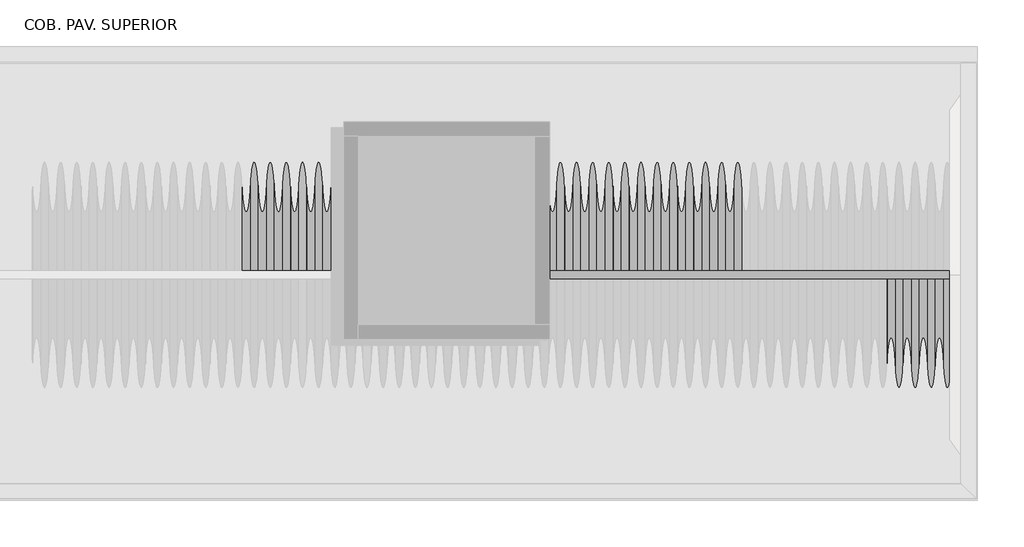
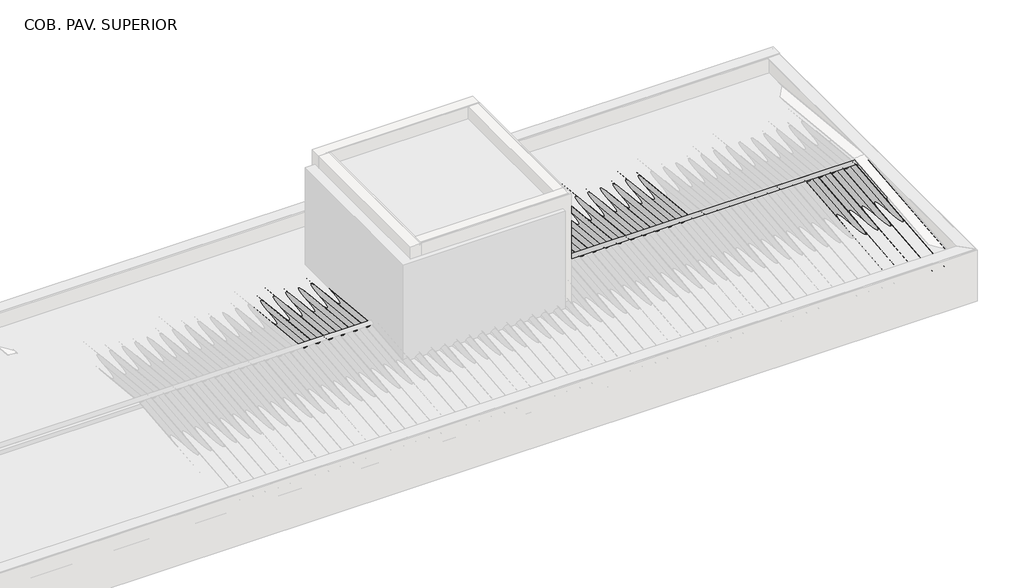
# One storey, part 7 of 8: 46 beams, 8 columns.
"""IFC4 building model written with IfcOpenShell, lengths in millimetres."""

import ifcopenshell
import ifcopenshell.guid

model = None  # the IFC model being written
_history = None  # IfcOwnerHistory: only IFC2X3 demands one
_inside = {}  # id of a spatial element -> (the spatial element, [elements in it])
_under = {}  # id of a project, library or spatial element -> (it, [spatial elements below it])
_declared = {}  # id of a project -> (the project, [libraries it declares])
_typed = {}  # id of a type object -> (the type object, [elements of that type])
_made_of = {}  # id of a material, layer set ... -> (it, [elements and type objects made of it])


def new_model(schema):
    """Start an empty IFC model of exactly this schema.

    Asked for "IFC4X3", IfcOpenShell would pick the latest addendum, in which some entities
    have other attributes; the version numbers below select the first issue.
    IFC2X3 requires an IfcOwnerHistory on every rooted entity: one is made here for all.
    """
    global model, _history
    if schema == "IFC4X3":
        model = ifcopenshell.file(schema_version=(4, 3, 0, 0))
    else:
        model = ifcopenshell.file(schema=schema)
    _inside.clear()
    _under.clear()
    _declared.clear()
    _typed.clear()
    _made_of.clear()
    _history = None
    if model.schema == "IFC2X3":
        org = make("IfcOrganization", Name="unknown")
        user = make(
            "IfcPersonAndOrganization",
            ThePerson=make("IfcPerson", FamilyName="unknown"),
            TheOrganization=org,
        )
        app = make(
            "IfcApplication",
            ApplicationDeveloper=org,
            Version="unknown",
            ApplicationFullName="unknown",
            ApplicationIdentifier="unknown",
        )
        _history = make(
            "IfcOwnerHistory",
            OwningUser=user,
            OwningApplication=app,
            ChangeAction="ADDED",
            CreationDate=0,
        )
    return model


def make(cls, **values):
    """One entity of the class cls with the attributes given. An attribute that is None is left unset."""
    return model.create_entity(
        cls, **{name: value for name, value in values.items() if value is not None}
    )


def rooted(cls, **values):
    """An entity with a GlobalId (a new one), such as an element, a storey or a relation."""
    return make(cls, GlobalId=ifcopenshell.guid.new(), OwnerHistory=_history, **values)


def si_unit(unit_type, name, prefix=None):
    """IfcSIUnit, for example si_unit("LENGTHUNIT", "METRE", prefix="MILLI")."""
    return make("IfcSIUnit", UnitType=unit_type, Prefix=prefix, Name=name)


def assignment(units):
    """IfcUnitAssignment: the units of a project."""
    return None if units is None else make("IfcUnitAssignment", Units=units)


def point(xyz):
    """IfcCartesianPoint."""
    return None if xyz is None else make("IfcCartesianPoint", Coordinates=xyz)


def direction(xyz):
    """IfcDirection."""
    return None if xyz is None else make("IfcDirection", DirectionRatios=xyz)


def frame(location, z_axis=None, x_axis=None):
    """IfcAxis2Placement3D, a coordinate frame: its origin and axes. An axis left out is left unset."""
    return make(
        "IfcAxis2Placement3D",
        Location=point(location),
        Axis=direction(z_axis),
        RefDirection=direction(x_axis),
    )


def frame_2d(location, x_axis=None):
    """IfcAxis2Placement2D, a coordinate frame in the plane: its origin and x axis."""
    return make(
        "IfcAxis2Placement2D", Location=point(location), RefDirection=direction(x_axis)
    )


def origin():
    """The frame at (0, 0, 0) with its axes left unset."""
    return frame((0.0, 0.0, 0.0))


def place(relative_to, where):
    """IfcLocalPlacement: puts the frame where relative to a parent placement (None: the world)."""
    return make(
        "IfcLocalPlacement", PlacementRelTo=relative_to, RelativePlacement=where
    )


def context(
    kind, dimensions, precision=None, world=None, true_north=None, identifier=None
):
    """IfcGeometricRepresentationContext, for example the 3D "Model" context."""
    return make(
        "IfcGeometricRepresentationContext",
        ContextIdentifier=identifier,
        ContextType=kind,
        CoordinateSpaceDimension=dimensions,
        Precision=precision,
        WorldCoordinateSystem=world,
        TrueNorth=true_north,
    )


def project(units=None, contexts=None):
    """IfcProject with its units and contexts."""
    return rooted(
        "IfcProject",
        Name="project",
        RepresentationContexts=contexts,
        UnitsInContext=assignment(units),
    )


def spatial(cls, under=None, at=None, **own):
    """A site, building, storey or space (cls), placed at a placement, below another one or the project."""
    s = rooted(cls, ObjectPlacement=at, **own)
    if under is not None:
        _under.setdefault(under.id(), (under, []))[1].append(s)
    return s


def polyline(points):
    """IfcPolyline through the points."""
    return make("IfcPolyline", Points=[point(p) for p in points])


def circle_curve(where, radius):
    """IfcCircle in the frame where."""
    return make("IfcCircle", Position=where, Radius=radius)


def trimmed(basis, trim1, trim2, sense, master):
    """IfcTrimmedCurve: the piece of a basis curve between two trims."""
    return make(
        "IfcTrimmedCurve",
        BasisCurve=basis,
        Trim1=trim1,
        Trim2=trim2,
        SenseAgreement=sense,
        MasterRepresentation=master,
    )


def segment(curve, same_sense, transition):
    """IfcCompositeCurveSegment."""
    return make(
        "IfcCompositeCurveSegment",
        Transition=transition,
        SameSense=same_sense,
        ParentCurve=curve,
    )


def composite_curve(segments, self_intersect=None):
    """IfcCompositeCurve: segments joined end to end."""
    return make("IfcCompositeCurve", Segments=segments, SelfIntersect=self_intersect)


def outline(outer, holes=None, kind="AREA"):
    """IfcArbitraryClosedProfileDef: a profile drawn as a closed curve; with holes, ...WithVoids."""
    if holes is None:
        return make("IfcArbitraryClosedProfileDef", ProfileType=kind, OuterCurve=outer)
    return make(
        "IfcArbitraryProfileDefWithVoids",
        ProfileType=kind,
        OuterCurve=outer,
        InnerCurves=holes,
    )


def extrude(swept, where, along, depth):
    """IfcExtrudedAreaSolid: the profile swept, set in the frame where, extruded along a direction by depth."""
    return make(
        "IfcExtrudedAreaSolid",
        SweptArea=swept,
        Position=where,
        ExtrudedDirection=direction(along),
        Depth=depth,
    )


def shape(context_of_items, identifier, shape_type, items):
    """IfcShapeRepresentation: the items that make up one representation, for example the "Body"."""
    return make(
        "IfcShapeRepresentation",
        ContextOfItems=context_of_items,
        RepresentationIdentifier=identifier,
        RepresentationType=shape_type,
        Items=items,
    )


def source(mapping_origin, context_of_items, identifier, shape_type, items):
    """IfcRepresentationMap: a shape defined once, which mapped items show again and again."""
    return make(
        "IfcRepresentationMap",
        MappingOrigin=mapping_origin,
        MappedRepresentation=shape(context_of_items, identifier, shape_type, items),
    )


def transform(
    local_origin,
    x_axis=None,
    y_axis=None,
    z_axis=None,
    scale=None,
    scale2=None,
    scale3=None,
    uniform=True,
):
    """IfcCartesianTransformationOperator3D, or its non-uniform kind. x_axis, y_axis, z_axis: its Axis1, 2, 3."""
    if uniform:
        return make(
            "IfcCartesianTransformationOperator3D",
            Axis1=direction(x_axis),
            Axis2=direction(y_axis),
            LocalOrigin=point(local_origin),
            Scale=scale,
            Axis3=direction(z_axis),
        )
    return make(
        "IfcCartesianTransformationOperator3DnonUniform",
        Axis1=direction(x_axis),
        Axis2=direction(y_axis),
        LocalOrigin=point(local_origin),
        Scale=scale,
        Axis3=direction(z_axis),
        Scale2=scale2,
        Scale3=scale3,
    )


def mapped(mapping_source, mapping_target):
    """IfcMappedItem: shows the shape of a source again, moved by a transform."""
    return make(
        "IfcMappedItem", MappingSource=mapping_source, MappingTarget=mapping_target
    )


def made_of(thing, what):
    """Note that an element or type object is made of a material, layer set ...; save() writes the relation."""
    if what is not None:
        _made_of.setdefault(what.id(), (what, []))[1].append(thing)
    return thing


def element(
    cls,
    number,
    at=None,
    inside=None,
    cuts=None,
    type_object=None,
    material=None,
    context=None,
    identifier="Body",
    shape_type=None,
    held_by="IfcProductDefinitionShape",
    body=None,
    shapes=None,
    **own,
):
    """One element of the class cls, such as IfcWall. Its Tag is "e" and its number.

    at: its placement. inside: the storey or other place that contains it. cuts: it is an
    opening in that element (IfcRelVoidsElement). A single representation is given by context,
    identifier, shape_type and body (its items); several are given by shapes. held_by: the class
    of the entity that holds the representations. save() writes the other relations.
    """
    e = rooted(cls, Tag="e%d" % number, ObjectPlacement=at, **own)
    if body is not None:
        shapes = [shape(context, identifier, shape_type, body)]
    if shapes is not None:
        e.Representation = make(held_by, Representations=shapes)
    if inside is not None:
        _inside.setdefault(inside.id(), (inside, []))[1].append(e)
    if cuts is not None:
        rooted(
            "IfcRelVoidsElement", RelatingBuildingElement=cuts, RelatedOpeningElement=e
        )
    if type_object is not None:
        _typed.setdefault(type_object.id(), (type_object, []))[1].append(e)
    return made_of(e, material)


def aggregate(whole, parts):
    """IfcRelAggregates: a whole, such as a stair, and the parts it consists of."""
    return rooted("IfcRelAggregates", RelatingObject=whole, RelatedObjects=parts)


def save(model, path):
    """Write the relations noted so far, then the file.

    IfcRelAggregates (storeys below a building ...), IfcRelContainedInSpatialStructure (elements
    in a storey), IfcRelDefinesByType, IfcRelAssociatesMaterial and IfcRelDeclares: one each for
    every whole, place, type object, material and project.
    """
    for whole, parts in _under.values():
        aggregate(whole, parts)
    for where, things in _inside.values():
        rooted(
            "IfcRelContainedInSpatialStructure",
            RelatedElements=things,
            RelatingStructure=where,
        )
    for kind, things in _typed.values():
        rooted("IfcRelDefinesByType", RelatedObjects=things, RelatingType=kind)
    for what, things in _made_of.values():
        rooted("IfcRelAssociatesMaterial", RelatedObjects=things, RelatingMaterial=what)
    for by, libraries in _declared.values():
        rooted("IfcRelDeclares", RelatingContext=by, RelatedDefinitions=libraries)
    model.write(path)


def beam_fe4ddbad(model_context):
    return source(origin(), model_context, "Body", "SweptSolid", [
        extrude(outline(polyline([(998.8971968, 30.0), (998.8971968, -30.0), (-998.8971974, -30.0), (-998.8971974, 30.0), (998.8971968, 30.0)])), frame((0.0, 0.0, -60.0), z_axis=(0.0, 0.0, 1.0), x_axis=(1.0, 0.0, 0.0)), (0.0, 0.0, 1.0), 120.0),
    ])


def beam_14fb2a3a(model_context):
    return source(origin(), model_context, "Body", "SweptSolid", [
        extrude(outline(polyline([(90.6640427, 30.0), (90.6640427, -30.0), (-90.6640427, -30.0), (-90.6640427, 30.0), (90.6640427, 30.0)])), frame((0.0, 0.0, -60.0), z_axis=(0.0, 0.0, 1.0), x_axis=(1.0, 0.0, 0.0)), (0.0, 0.0, 1.0), 120.0),
    ])


def beam_531541e1(model_context):
    return source(origin(), model_context, "Body", "SweptSolid", [
        extrude(outline(polyline([(789.5608169, 30.0), (789.5608169, -30.0), (-789.5608169, -30.0), (-789.5608169, 30.0), (789.5608169, 30.0)])), frame((0.0, 0.0, -60.0), z_axis=(0.0, 0.0, 1.0), x_axis=(1.0, 0.0, 0.0)), (0.0, 0.0, 1.0), 120.0),
    ])


def cumeeira_telha_ondulada_fibrocimento_e54732c7(model_context):
    return source(origin(), model_context, "Body", "SweptSolid", [
        extrude(outline(composite_curve([segment(polyline([(58.3970135, 42.4437972), (53.9055884, 40.2467307)]), True, "CONTINUOUS"), segment(trimmed(circle_curve(frame_2d((-1.6029865, 13.0936483)), 61.7939461), [point((53.9055884, 40.2467307))], [point((-57.1115615, 40.2467307))], True, "CARTESIAN"), True, "CONTINUOUS"), segment(polyline([(-57.1115615, 40.2467307), (-61.6029865, 42.4437972)]), True, "CONTINUOUS"), segment(trimmed(circle_curve(frame_2d((-1.6029865, 13.0936483)), 66.7939461), [point((-61.6029865, 42.4437972))], [point((58.3970135, 42.4437972))], False, "CARTESIAN"), True, "CONTINUOUS")], self_intersect=False)), frame((-3133.4781794, 0.0, 0.0), z_axis=(1.0, 0.0, 0.0), x_axis=(0.0, 1.0, 0.0)), (0.0, 0.0, 1.0), 6266.9563589),
    ])


def telha_ondulada_fibrocimento_963230a9(model_context):
    return source(origin(), model_context, "Body", "SweptSolid", [
        extrude(outline(composite_curve([segment(trimmed(circle_curve(frame_2d((68.3970135, 71.7939461)), 66.7939461), [point((8.3970135, 42.4437972))], [point((128.3970135, 42.4437972))], True, "CARTESIAN"), True, "CONTINUOUS"), segment(polyline([(128.3970135, 42.4437972), (132.8884385, 40.2467307)]), True, "CONTINUOUS"), segment(trimmed(circle_curve(frame_2d((68.3970135, 71.7939461)), 71.7939461), [point((132.8884385, 40.2467307))], [point((3.9055884, 40.2467307))], False, "CARTESIAN"), True, "CONTINUOUS"), segment(trimmed(circle_curve(frame_2d((-51.6029865, 13.0936483)), 61.7939461), [point((3.9055884, 40.2467307))], [point((-107.1115615, 40.2467307))], True, "CARTESIAN"), True, "CONTINUOUS"), segment(polyline([(-107.1115615, 40.2467307), (-111.6029865, 42.4437972)]), True, "CONTINUOUS"), segment(trimmed(circle_curve(frame_2d((-51.6029865, 13.0936483)), 66.7939461), [point((-111.6029865, 42.4437972))], [point((8.3970135, 42.4437972))], False, "CARTESIAN"), True, "CONTINUOUS")], self_intersect=False)), frame((-362.9289365, 0.0, 0.0), z_axis=(1.0, 0.0, 0.0), x_axis=(0.0, 1.0, 0.0)), (0.0, 0.0, 1.0), 725.8578731),
    ])


def viga_cumeeira_6x16cm_e360fa9d(model_context):
    return source(origin(), model_context, "Body", "SweptSolid", [
        extrude(outline(polyline([(3133.5, 30.0), (3133.5, -30.0), (-3133.5, -30.0), (-3133.5, 30.0), (3133.5, 30.0)])), frame((0.0, 0.0, -80.0), z_axis=(0.0, 0.0, 1.0), x_axis=(1.0, 0.0, 0.0)), (0.0, 0.0, 1.0), 160.0),
    ])


def column_6c15bf79(model_context):
    return source(origin(), model_context, "Body", "SweptSolid", [
        extrude(outline(polyline([(30.0, 80.0), (30.0, -80.0), (-30.0, -80.0), (-30.0, 80.0), (30.0, 80.0)])), frame((0.0, 0.0, 6710.0), z_axis=(0.0, 0.0, 1.0), x_axis=(1.0, 0.0, 0.0)), (0.0, 0.0, 1.0), 467.5),
    ])


def column_910cb117(model_context):
    return source(origin(), model_context, "Body", "SweptSolid", [
        extrude(outline(polyline([(30.0, 80.0), (30.0, -80.0), (-30.0, -80.0), (-30.0, 80.0), (30.0, 80.0)])), frame((0.0, 0.0, 6710.0), z_axis=(0.0, 0.0, 1.0), x_axis=(1.0, 0.0, 0.0)), (0.0, 0.0, 1.0), 371.3),
    ])


def column_42eef9f8(model_context):
    return source(origin(), model_context, "Body", "SweptSolid", [
        extrude(outline(polyline([(30.0, 80.0), (30.0, -80.0), (-30.0, -80.0), (-30.0, 80.0), (30.0, 80.0)])), frame((0.0, 0.0, 6710.0), z_axis=(0.0, 0.0, 1.0), x_axis=(1.0, 0.0, 0.0)), (0.0, 0.0, 1.0), 227.1),
    ])


model = new_model("IFC4")

# Units and contexts
model_context = context("Model", 3, world=origin())
ifc_project = project(units=[si_unit("LENGTHUNIT", "METRE", prefix="MILLI")], contexts=[model_context])

# Site, building, storey
site = spatial("IfcSite", under=ifc_project)
building = spatial("IfcBuilding", under=site)
storey = spatial("IfcBuildingStorey", under=building, Name="COB. PAV. SUPERIOR", Elevation=6650.0)

# Beams
placement = place(None, origin())
beam_shape = beam_fe4ddbad(model_context)
element("IfcBeam", 1, ObjectType="Madeira de lei : Berço 6x12cm", at=placement, inside=storey, context=model_context, shape_type="MappedRepresentation", body=[
    mapped(beam_shape, transform((5549.6158904, -7777.6209418, 6680.0), x_axis=(1.0, 0.0, 0.0), y_axis=(0.0, 0.0, -1.0), z_axis=(0.0, 1.0, 0.0))),
])
element("IfcBeam", 2, ObjectType="Madeira de lei : Berço 6x12cm", at=placement, inside=storey, context=model_context, shape_type="MappedRepresentation", body=[
    mapped(beam_shape, transform((5549.6158904, -6365.3711004, 6680.0), x_axis=(1.0, 0.0, 0.0), y_axis=(0.0, 0.0, -1.0), z_axis=(0.0, 1.0, 0.0))),
])
element("IfcBeam", 3, ObjectType="Madeira de lei : Berço 6x12cm", at=placement, inside=storey, context=model_context, shape_type="MappedRepresentation", body=[
    mapped(beam_shape, transform((7547.4102853, -7777.6209418, 6680.0), x_axis=(1.0, 0.0, 0.0), y_axis=(0.0, 0.0, -1.0), z_axis=(0.0, 1.0, 0.0))),
])
element("IfcBeam", 4, ObjectType="Madeira de lei : Berço 6x12cm", at=placement, inside=storey, context=model_context, shape_type="MappedRepresentation", body=[
    mapped(beam_shape, transform((248.5822594, -7777.6209418, 6680.0), x_axis=(1.0, 0.0, 0.0), y_axis=(0.0, 0.0, -1.0), z_axis=(0.0, 1.0, 0.0))),
])
element("IfcBeam", 5, ObjectType="Madeira de lei : Berço 6x12cm", at=placement, inside=storey, context=model_context, shape_type="MappedRepresentation", body=[
    mapped(beam_shape, transform((248.5822594, -6365.3711004, 6680.0), x_axis=(1.0, 0.0, 0.0), y_axis=(0.0, 0.0, -1.0), z_axis=(0.0, 1.0, 0.0))),
])
element("IfcBeam", 6, ObjectType="Madeira de lei : Berço 6x12cm", at=placement, inside=storey, context=model_context, shape_type="MappedRepresentation", body=[
    mapped(beam_shape, transform((2246.3766557, -4923.3211004, 6680.0), x_axis=(1.0, 0.0, 0.0), y_axis=(0.0, 0.0, -1.0), z_axis=(0.0, 1.0, 0.0))),
])
element("IfcBeam", 7, ObjectType="Madeira de lei : Berço 6x12cm", at=placement, inside=storey, context=model_context, shape_type="MappedRepresentation", body=[
    mapped(beam_shape, transform((248.5822615, -4923.3211004, 6680.0), x_axis=(1.0, 0.0, 0.0), y_axis=(0.0, 0.0, -1.0), z_axis=(0.0, 1.0, 0.0))),
])
beam_2_shape = beam_14fb2a3a(model_context)
element("IfcBeam", 8, ObjectType="Madeira de lei : Berço 6x12cm", at=placement, inside=storey, context=model_context, shape_type="MappedRepresentation", body=[
    mapped(beam_2_shape, transform((1338.1434995, -7777.6209418, 6680.0), x_axis=(1.0, 0.0, 0.0), y_axis=(0.0, 0.0, -1.0), z_axis=(0.0, 1.0, 0.0))),
])
element("IfcBeam", 9, ObjectType="Madeira de lei : Berço 6x12cm", at=placement, inside=storey, context=model_context, shape_type="MappedRepresentation", body=[
    mapped(beam_2_shape, transform((1338.1434995, -6365.3711004, 6680.0), x_axis=(1.0, 0.0, 0.0), y_axis=(0.0, 0.0, -1.0), z_axis=(0.0, 1.0, 0.0))),
])
beam_3_shape = beam_531541e1(model_context)
element("IfcBeam", 10, ObjectType="Madeira de lei : Berço 6x12cm", at=placement, inside=storey, context=model_context, shape_type="MappedRepresentation", body=[
    mapped(beam_3_shape, transform((10028.217853, -9189.768869, 6680.0), x_axis=(1.0, 0.0, 0.0), y_axis=(0.0, 0.0, -1.0), z_axis=(0.0, 1.0, 0.0))),
])
cumeeira_telha_ondulada_fibrocimento_shape = cumeeira_telha_ondulada_fibrocimento_e54732c7(model_context)
element("IfcBeam", 11, ObjectType="Cumeeira Telha Ondulada : Fibrocimento", at=placement, inside=storey, context=model_context, shape_type="MappedRepresentation", body=[
    mapped(cumeeira_telha_ondulada_fibrocimento_shape, transform((7684.2405136, -7777.6209418, 7375.6251229), x_axis=(-1.0, 0.0, 0.0), y_axis=(0.0, -1.0, 0.0), z_axis=(0.0, 0.0, 1.0))),
])
element("IfcBeam", 12, ObjectType="Telha Ondulada : Fibrocimento", at=placement, inside=storey, context=model_context, shape_type="SweptSolid", body=[
    extrude(outline(composite_curve([segment(trimmed(circle_curve(frame_2d((0.0, 66.7939461)), 66.7939461), [point((29.3501489, 6.7939461))], [point((29.3501489, 126.7939461))], True, "CARTESIAN"), True, "CONTINUOUS"), segment(polyline([(29.3501489, 126.7939461), (31.5472154, 131.2853711)]), True, "CONTINUOUS"), segment(trimmed(circle_curve(frame_2d((0.0, 66.7939461)), 71.7939461), [point((31.5472154, 131.2853711))], [point((31.5472154, 2.3025211))], False, "CARTESIAN"), True, "CONTINUOUS"), segment(trimmed(circle_curve(frame_2d((58.7002978, -53.2060539)), 61.7939461), [point((31.5472154, 2.3025211))], [point((31.5472154, -108.7146289))], True, "CARTESIAN"), True, "CONTINUOUS"), segment(polyline([(31.5472154, -108.7146289), (29.3501489, -113.2060539)]), True, "CONTINUOUS"), segment(trimmed(circle_curve(frame_2d((58.7002978, -53.2060539)), 66.7939461), [point((29.3501489, -113.2060539))], [point((29.3501489, 6.7939461))], False, "CARTESIAN"), True, "CONTINUOUS")], self_intersect=False)), frame((9796.7156257, -10831.9594023, 7106.8215886), z_axis=(0.0, 0.9950371902099894, 0.09950371902099749), x_axis=(0.0, 0.09950371902099749, -0.9950371902099894)), (0.0, 0.0, 1.0), 3060.4439799),
])
element("IfcBeam", 13, ObjectType="Telha Ondulada : Fibrocimento", at=placement, inside=storey, context=model_context, shape_type="SweptSolid", body=[
    extrude(outline(composite_curve([segment(trimmed(circle_curve(frame_2d((0.0, 66.7939461)), 66.7939461), [point((29.3501489, 6.7939461))], [point((29.3501489, 126.7939461))], True, "CARTESIAN"), True, "CONTINUOUS"), segment(polyline([(29.3501489, 126.7939461), (31.5472154, 131.2853711)]), True, "CONTINUOUS"), segment(trimmed(circle_curve(frame_2d((0.0, 66.7939461)), 71.7939461), [point((31.5472154, 131.2853711))], [point((31.5472154, 2.3025211))], False, "CARTESIAN"), True, "CONTINUOUS"), segment(trimmed(circle_curve(frame_2d((58.7002978, -53.2060539)), 61.7939461), [point((31.5472154, 2.3025211))], [point((31.5472154, -108.7146289))], True, "CARTESIAN"), True, "CONTINUOUS"), segment(polyline([(31.5472154, -108.7146289), (29.3501489, -113.2060539)]), True, "CONTINUOUS"), segment(trimmed(circle_curve(frame_2d((58.7002978, -53.2060539)), 66.7939461), [point((29.3501489, -113.2060539))], [point((29.3501489, 6.7939461))], False, "CARTESIAN"), True, "CONTINUOUS")], self_intersect=False)), frame((10041.2156257, -10831.9594023, 7106.8215886), z_axis=(0.0, 0.9950371902099894, 0.09950371902099749), x_axis=(0.0, 0.09950371902099749, -0.9950371902099894)), (0.0, 0.0, 1.0), 3060.4439799),
])
element("IfcBeam", 14, ObjectType="Telha Ondulada : Fibrocimento", at=placement, inside=storey, context=model_context, shape_type="SweptSolid", body=[
    extrude(outline(composite_curve([segment(trimmed(circle_curve(frame_2d((0.0, 66.7939461)), 66.7939461), [point((29.3501489, 6.7939461))], [point((29.3501489, 126.7939461))], True, "CARTESIAN"), True, "CONTINUOUS"), segment(polyline([(29.3501489, 126.7939461), (31.5472154, 131.2853711)]), True, "CONTINUOUS"), segment(trimmed(circle_curve(frame_2d((0.0, 66.7939461)), 71.7939461), [point((31.5472154, 131.2853711))], [point((31.5472154, 2.3025211))], False, "CARTESIAN"), True, "CONTINUOUS"), segment(trimmed(circle_curve(frame_2d((58.7002978, -53.2060539)), 61.7939461), [point((31.5472154, 2.3025211))], [point((31.5472154, -108.7146289))], True, "CARTESIAN"), True, "CONTINUOUS"), segment(polyline([(31.5472154, -108.7146289), (29.3501489, -113.2060539)]), True, "CONTINUOUS"), segment(trimmed(circle_curve(frame_2d((58.7002978, -53.2060539)), 66.7939461), [point((29.3501489, -113.2060539))], [point((29.3501489, 6.7939461))], False, "CARTESIAN"), True, "CONTINUOUS")], self_intersect=False)), frame((10285.7156257, -10831.9594023, 7106.8215886), z_axis=(0.0, 0.9950371902099894, 0.09950371902099749), x_axis=(0.0, 0.09950371902099749, -0.9950371902099894)), (0.0, 0.0, 1.0), 3060.4439799),
])
element("IfcBeam", 15, ObjectType="Telha Ondulada : Fibrocimento", at=placement, inside=storey, context=model_context, shape_type="SweptSolid", body=[
    extrude(outline(composite_curve([segment(trimmed(circle_curve(frame_2d((0.0, 66.7939461)), 66.7939461), [point((29.3501489, 6.7939461))], [point((29.3501489, 126.7939461))], True, "CARTESIAN"), True, "CONTINUOUS"), segment(polyline([(29.3501489, 126.7939461), (31.5472154, 131.2853711)]), True, "CONTINUOUS"), segment(trimmed(circle_curve(frame_2d((0.0, 66.7939461)), 71.7939461), [point((31.5472154, 131.2853711))], [point((31.5472154, 2.3025211))], False, "CARTESIAN"), True, "CONTINUOUS"), segment(trimmed(circle_curve(frame_2d((58.7002978, -53.2060539)), 61.7939461), [point((31.5472154, 2.3025211))], [point((31.5472154, -108.7146289))], True, "CARTESIAN"), True, "CONTINUOUS"), segment(polyline([(31.5472154, -108.7146289), (29.3501489, -113.2060539)]), True, "CONTINUOUS"), segment(trimmed(circle_curve(frame_2d((58.7002978, -53.2060539)), 66.7939461), [point((29.3501489, -113.2060539))], [point((29.3501489, 6.7939461))], False, "CARTESIAN"), True, "CONTINUOUS")], self_intersect=False)), frame((10530.2156257, -10831.9594023, 7106.8215886), z_axis=(0.0, 0.9950371902099894, 0.09950371902099749), x_axis=(0.0, 0.09950371902099749, -0.9950371902099894)), (0.0, 0.0, 1.0), 3060.4439799),
])
element("IfcBeam", 16, ObjectType="Telha Ondulada : Fibrocimento", at=placement, inside=storey, context=model_context, shape_type="SweptSolid", body=[
    extrude(outline(composite_curve([segment(trimmed(circle_curve(frame_2d((0.0, 66.7939461)), 66.7939461), [point((29.3501489, 6.7939461))], [point((29.3501489, 126.7939461))], True, "CARTESIAN"), True, "CONTINUOUS"), segment(polyline([(29.3501489, 126.7939461), (31.5472154, 131.2853711)]), True, "CONTINUOUS"), segment(trimmed(circle_curve(frame_2d((0.0, 66.7939461)), 71.7939461), [point((31.5472154, 131.2853711))], [point((31.5472154, 2.3025211))], False, "CARTESIAN"), True, "CONTINUOUS"), segment(trimmed(circle_curve(frame_2d((58.7002978, -53.2060539)), 61.7939461), [point((31.5472154, 2.3025211))], [point((31.5472154, -108.7146289))], True, "CARTESIAN"), True, "CONTINUOUS"), segment(polyline([(31.5472154, -108.7146289), (29.3501489, -113.2060539)]), True, "CONTINUOUS"), segment(trimmed(circle_curve(frame_2d((58.7002978, -53.2060539)), 66.7939461), [point((29.3501489, -113.2060539))], [point((29.3501489, 6.7939461))], False, "CARTESIAN"), True, "CONTINUOUS")], self_intersect=False)), frame((10774.7156257, -10831.9594023, 7106.8215886), z_axis=(0.0, 0.9950371902099894, 0.09950371902099749), x_axis=(0.0, 0.09950371902099749, -0.9950371902099894)), (0.0, 0.0, 1.0), 3060.4439799),
])
element("IfcBeam", 17, ObjectType="Telha Ondulada : Fibrocimento", at=placement, inside=storey, context=model_context, shape_type="SweptSolid", body=[
    extrude(outline(composite_curve([segment(trimmed(circle_curve(frame_2d((-58.7002978, -53.2060539)), 66.7939461), [point((-29.3501489, 6.7939461))], [point((-29.3501489, -113.2060539))], False, "CARTESIAN"), True, "CONTINUOUS"), segment(polyline([(-29.3501489, -113.2060539), (-31.5472154, -108.7146289)]), True, "CONTINUOUS"), segment(trimmed(circle_curve(frame_2d((-58.7002978, -53.2060539)), 61.7939461), [point((-31.5472154, -108.7146289))], [point((-31.5472154, 2.3025211))], True, "CARTESIAN"), True, "CONTINUOUS"), segment(trimmed(circle_curve(frame_2d((0.0, 66.7939461)), 71.7939461), [point((-31.5472154, 2.3025211))], [point((-31.5472154, 131.2853711))], False, "CARTESIAN"), True, "CONTINUOUS"), segment(polyline([(-31.5472154, 131.2853711), (-29.3501489, 126.7939461)]), True, "CONTINUOUS"), segment(trimmed(circle_curve(frame_2d((0.0, 66.7939461)), 66.7939461), [point((-29.3501489, 126.7939461))], [point((-29.3501489, 6.7939461))], True, "CARTESIAN"), True, "CONTINUOUS")], self_intersect=False)), frame((16.7156257, -4723.1805671, 7106.8215886), z_axis=(0.0, -0.9950371902099893, 0.09950371902099796), x_axis=(0.0, 0.09950371902099796, 0.9950371902099893)), (0.0, 0.0, 1.0), 3060.4439799),
])
element("IfcBeam", 18, ObjectType="Telha Ondulada : Fibrocimento", at=placement, inside=storey, context=model_context, shape_type="SweptSolid", body=[
    extrude(outline(composite_curve([segment(trimmed(circle_curve(frame_2d((-58.7002978, -53.2060539)), 66.7939461), [point((-29.3501489, 6.7939461))], [point((-29.3501489, -113.2060539))], False, "CARTESIAN"), True, "CONTINUOUS"), segment(polyline([(-29.3501489, -113.2060539), (-31.5472154, -108.7146289)]), True, "CONTINUOUS"), segment(trimmed(circle_curve(frame_2d((-58.7002978, -53.2060539)), 61.7939461), [point((-31.5472154, -108.7146289))], [point((-31.5472154, 2.3025211))], True, "CARTESIAN"), True, "CONTINUOUS"), segment(trimmed(circle_curve(frame_2d((0.0, 66.7939461)), 71.7939461), [point((-31.5472154, 2.3025211))], [point((-31.5472154, 131.2853711))], False, "CARTESIAN"), True, "CONTINUOUS"), segment(polyline([(-31.5472154, 131.2853711), (-29.3501489, 126.7939461)]), True, "CONTINUOUS"), segment(trimmed(circle_curve(frame_2d((0.0, 66.7939461)), 66.7939461), [point((-29.3501489, 126.7939461))], [point((-29.3501489, 6.7939461))], True, "CARTESIAN"), True, "CONTINUOUS")], self_intersect=False)), frame((261.2156257, -4723.1805671, 7106.8215886), z_axis=(0.0, -0.9950371902099893, 0.09950371902099796), x_axis=(0.0, 0.09950371902099796, 0.9950371902099893)), (0.0, 0.0, 1.0), 3060.4439799),
])
element("IfcBeam", 19, ObjectType="Telha Ondulada : Fibrocimento", at=placement, inside=storey, context=model_context, shape_type="SweptSolid", body=[
    extrude(outline(composite_curve([segment(trimmed(circle_curve(frame_2d((-58.7002978, -53.2060539)), 66.7939461), [point((-29.3501489, 6.7939461))], [point((-29.3501489, -113.2060539))], False, "CARTESIAN"), True, "CONTINUOUS"), segment(polyline([(-29.3501489, -113.2060539), (-31.5472154, -108.7146289)]), True, "CONTINUOUS"), segment(trimmed(circle_curve(frame_2d((-58.7002978, -53.2060539)), 61.7939461), [point((-31.5472154, -108.7146289))], [point((-31.5472154, 2.3025211))], True, "CARTESIAN"), True, "CONTINUOUS"), segment(trimmed(circle_curve(frame_2d((0.0, 66.7939461)), 71.7939461), [point((-31.5472154, 2.3025211))], [point((-31.5472154, 131.2853711))], False, "CARTESIAN"), True, "CONTINUOUS"), segment(polyline([(-31.5472154, 131.2853711), (-29.3501489, 126.7939461)]), True, "CONTINUOUS"), segment(trimmed(circle_curve(frame_2d((0.0, 66.7939461)), 66.7939461), [point((-29.3501489, 126.7939461))], [point((-29.3501489, 6.7939461))], True, "CARTESIAN"), True, "CONTINUOUS")], self_intersect=False)), frame((505.7156257, -4723.1805671, 7106.8215886), z_axis=(0.0, -0.9950371902099893, 0.09950371902099796), x_axis=(0.0, 0.09950371902099796, 0.9950371902099893)), (0.0, 0.0, 1.0), 3060.4439799),
])
element("IfcBeam", 20, ObjectType="Telha Ondulada : Fibrocimento", at=placement, inside=storey, context=model_context, shape_type="SweptSolid", body=[
    extrude(outline(composite_curve([segment(trimmed(circle_curve(frame_2d((-58.7002978, -53.2060539)), 66.7939461), [point((-29.3501489, 6.7939461))], [point((-29.3501489, -113.2060539))], False, "CARTESIAN"), True, "CONTINUOUS"), segment(polyline([(-29.3501489, -113.2060539), (-31.5472154, -108.7146289)]), True, "CONTINUOUS"), segment(trimmed(circle_curve(frame_2d((-58.7002978, -53.2060539)), 61.7939461), [point((-31.5472154, -108.7146289))], [point((-31.5472154, 2.3025211))], True, "CARTESIAN"), True, "CONTINUOUS"), segment(trimmed(circle_curve(frame_2d((0.0, 66.7939461)), 71.7939461), [point((-31.5472154, 2.3025211))], [point((-31.5472154, 131.2853711))], False, "CARTESIAN"), True, "CONTINUOUS"), segment(polyline([(-31.5472154, 131.2853711), (-29.3501489, 126.7939461)]), True, "CONTINUOUS"), segment(trimmed(circle_curve(frame_2d((0.0, 66.7939461)), 66.7939461), [point((-29.3501489, 126.7939461))], [point((-29.3501489, 6.7939461))], True, "CARTESIAN"), True, "CONTINUOUS")], self_intersect=False)), frame((750.2156257, -4723.1805671, 7106.8215886), z_axis=(0.0, -0.9950371902099893, 0.09950371902099796), x_axis=(0.0, 0.09950371902099796, 0.9950371902099893)), (0.0, 0.0, 1.0), 3060.4439799),
])
element("IfcBeam", 21, ObjectType="Telha Ondulada : Fibrocimento", at=placement, inside=storey, context=model_context, shape_type="SweptSolid", body=[
    extrude(outline(composite_curve([segment(trimmed(circle_curve(frame_2d((-58.7002978, -53.2060539)), 66.7939461), [point((-29.3501489, 6.7939461))], [point((-29.3501489, -113.2060539))], False, "CARTESIAN"), True, "CONTINUOUS"), segment(polyline([(-29.3501489, -113.2060539), (-31.5472154, -108.7146289)]), True, "CONTINUOUS"), segment(trimmed(circle_curve(frame_2d((-58.7002978, -53.2060539)), 61.7939461), [point((-31.5472154, -108.7146289))], [point((-31.5472154, 2.3025211))], True, "CARTESIAN"), True, "CONTINUOUS"), segment(trimmed(circle_curve(frame_2d((0.0, 66.7939461)), 71.7939461), [point((-31.5472154, 2.3025211))], [point((-31.5472154, 131.2853711))], False, "CARTESIAN"), True, "CONTINUOUS"), segment(polyline([(-31.5472154, 131.2853711), (-29.3501489, 126.7939461)]), True, "CONTINUOUS"), segment(trimmed(circle_curve(frame_2d((0.0, 66.7939461)), 66.7939461), [point((-29.3501489, 126.7939461))], [point((-29.3501489, 6.7939461))], True, "CARTESIAN"), True, "CONTINUOUS")], self_intersect=False)), frame((994.7156257, -4723.1805671, 7106.8215886), z_axis=(0.0, -0.9950371902099893, 0.09950371902099796), x_axis=(0.0, 0.09950371902099796, 0.9950371902099893)), (0.0, 0.0, 1.0), 3060.4439799),
])
element("IfcBeam", 22, ObjectType="Telha Ondulada : Fibrocimento", at=placement, inside=storey, context=model_context, shape_type="SweptSolid", body=[
    extrude(outline(composite_curve([segment(trimmed(circle_curve(frame_2d((-58.7002978, -53.2060539)), 66.7939461), [point((-29.3501489, 6.7939461))], [point((-29.3501489, -113.2060539))], False, "CARTESIAN"), True, "CONTINUOUS"), segment(polyline([(-29.3501489, -113.2060539), (-31.5472154, -108.7146289)]), True, "CONTINUOUS"), segment(trimmed(circle_curve(frame_2d((-58.7002978, -53.2060539)), 61.7939461), [point((-31.5472154, -108.7146289))], [point((-31.5472154, 2.3025211))], True, "CARTESIAN"), True, "CONTINUOUS"), segment(trimmed(circle_curve(frame_2d((0.0, 66.7939461)), 71.7939461), [point((-31.5472154, 2.3025211))], [point((-31.5472154, 131.2853711))], False, "CARTESIAN"), True, "CONTINUOUS"), segment(polyline([(-31.5472154, 131.2853711), (-29.3501489, 126.7939461)]), True, "CONTINUOUS"), segment(trimmed(circle_curve(frame_2d((0.0, 66.7939461)), 66.7939461), [point((-29.3501489, 126.7939461))], [point((-29.3501489, 6.7939461))], True, "CARTESIAN"), True, "CONTINUOUS")], self_intersect=False)), frame((1239.2156257, -4723.1805671, 7106.8215886), z_axis=(0.0, -0.9950371902099893, 0.09950371902099796), x_axis=(0.0, 0.09950371902099796, 0.9950371902099893)), (0.0, 0.0, 1.0), 3060.4439799),
])
element("IfcBeam", 23, ObjectType="Telha Ondulada : Fibrocimento", at=placement, inside=storey, context=model_context, shape_type="SweptSolid", body=[
    extrude(outline(composite_curve([segment(trimmed(circle_curve(frame_2d((-58.7002978, -53.2060539)), 66.7939461), [point((-29.3501489, 6.7939461))], [point((-29.3501489, -113.2060539))], False, "CARTESIAN"), True, "CONTINUOUS"), segment(polyline([(-29.3501489, -113.2060539), (-31.5472154, -108.7146289)]), True, "CONTINUOUS"), segment(trimmed(circle_curve(frame_2d((-58.7002978, -53.2060539)), 61.7939461), [point((-31.5472154, -108.7146289))], [point((-31.5472154, 2.3025211))], True, "CARTESIAN"), True, "CONTINUOUS"), segment(trimmed(circle_curve(frame_2d((0.0, 66.7939461)), 71.7939461), [point((-31.5472154, 2.3025211))], [point((-31.5472154, 131.2853711))], False, "CARTESIAN"), True, "CONTINUOUS"), segment(polyline([(-31.5472154, 131.2853711), (-29.3501489, 126.7939461)]), True, "CONTINUOUS"), segment(trimmed(circle_curve(frame_2d((0.0, 66.7939461)), 66.7939461), [point((-29.3501489, 126.7939461))], [point((-29.3501489, 6.7939461))], True, "CARTESIAN"), True, "CONTINUOUS")], self_intersect=False)), frame((4662.2156257, -4723.1805671, 7106.8215886), z_axis=(0.0, -0.9950371902099893, 0.09950371902099783), x_axis=(0.0, 0.09950371902099783, 0.9950371902099893)), (0.0, 0.0, 1.0), 3060.4439799),
])
element("IfcBeam", 24, ObjectType="Telha Ondulada : Fibrocimento", at=placement, inside=storey, context=model_context, shape_type="SweptSolid", body=[
    extrude(outline(composite_curve([segment(trimmed(circle_curve(frame_2d((-58.7002978, -53.2060539)), 66.7939461), [point((-29.3501489, 6.7939461))], [point((-29.3501489, -113.2060539))], False, "CARTESIAN"), True, "CONTINUOUS"), segment(polyline([(-29.3501489, -113.2060539), (-31.5472154, -108.7146289)]), True, "CONTINUOUS"), segment(trimmed(circle_curve(frame_2d((-58.7002978, -53.2060539)), 61.7939461), [point((-31.5472154, -108.7146289))], [point((-31.5472154, 2.3025211))], True, "CARTESIAN"), True, "CONTINUOUS"), segment(trimmed(circle_curve(frame_2d((0.0, 66.7939461)), 71.7939461), [point((-31.5472154, 2.3025211))], [point((-31.5472154, 131.2853711))], False, "CARTESIAN"), True, "CONTINUOUS"), segment(polyline([(-31.5472154, 131.2853711), (-29.3501489, 126.7939461)]), True, "CONTINUOUS"), segment(trimmed(circle_curve(frame_2d((0.0, 66.7939461)), 66.7939461), [point((-29.3501489, 126.7939461))], [point((-29.3501489, 6.7939461))], True, "CARTESIAN"), True, "CONTINUOUS")], self_intersect=False)), frame((4906.7156257, -4723.1805671, 7106.8215886), z_axis=(0.0, -0.9950371902099893, 0.09950371902099783), x_axis=(0.0, 0.09950371902099783, 0.9950371902099893)), (0.0, 0.0, 1.0), 3060.4439799),
])
element("IfcBeam", 25, ObjectType="Telha Ondulada : Fibrocimento", at=placement, inside=storey, context=model_context, shape_type="SweptSolid", body=[
    extrude(outline(composite_curve([segment(trimmed(circle_curve(frame_2d((-58.7002978, -53.2060539)), 66.7939461), [point((-29.3501489, 6.7939461))], [point((-29.3501489, -113.2060539))], False, "CARTESIAN"), True, "CONTINUOUS"), segment(polyline([(-29.3501489, -113.2060539), (-31.5472154, -108.7146289)]), True, "CONTINUOUS"), segment(trimmed(circle_curve(frame_2d((-58.7002978, -53.2060539)), 61.7939461), [point((-31.5472154, -108.7146289))], [point((-31.5472154, 2.3025211))], True, "CARTESIAN"), True, "CONTINUOUS"), segment(trimmed(circle_curve(frame_2d((0.0, 66.7939461)), 71.7939461), [point((-31.5472154, 2.3025211))], [point((-31.5472154, 131.2853711))], False, "CARTESIAN"), True, "CONTINUOUS"), segment(polyline([(-31.5472154, 131.2853711), (-29.3501489, 126.7939461)]), True, "CONTINUOUS"), segment(trimmed(circle_curve(frame_2d((0.0, 66.7939461)), 66.7939461), [point((-29.3501489, 126.7939461))], [point((-29.3501489, 6.7939461))], True, "CARTESIAN"), True, "CONTINUOUS")], self_intersect=False)), frame((5151.2156257, -4723.1805671, 7106.8215886), z_axis=(0.0, -0.9950371902099893, 0.09950371902099783), x_axis=(0.0, 0.09950371902099783, 0.9950371902099893)), (0.0, 0.0, 1.0), 3060.4439799),
])
element("IfcBeam", 26, ObjectType="Telha Ondulada : Fibrocimento", at=placement, inside=storey, context=model_context, shape_type="SweptSolid", body=[
    extrude(outline(composite_curve([segment(trimmed(circle_curve(frame_2d((-58.7002978, -53.2060539)), 66.7939461), [point((-29.3501489, 6.7939461))], [point((-29.3501489, -113.2060539))], False, "CARTESIAN"), True, "CONTINUOUS"), segment(polyline([(-29.3501489, -113.2060539), (-31.5472154, -108.7146289)]), True, "CONTINUOUS"), segment(trimmed(circle_curve(frame_2d((-58.7002978, -53.2060539)), 61.7939461), [point((-31.5472154, -108.7146289))], [point((-31.5472154, 2.3025211))], True, "CARTESIAN"), True, "CONTINUOUS"), segment(trimmed(circle_curve(frame_2d((0.0, 66.7939461)), 71.7939461), [point((-31.5472154, 2.3025211))], [point((-31.5472154, 131.2853711))], False, "CARTESIAN"), True, "CONTINUOUS"), segment(polyline([(-31.5472154, 131.2853711), (-29.3501489, 126.7939461)]), True, "CONTINUOUS"), segment(trimmed(circle_curve(frame_2d((0.0, 66.7939461)), 66.7939461), [point((-29.3501489, 126.7939461))], [point((-29.3501489, 6.7939461))], True, "CARTESIAN"), True, "CONTINUOUS")], self_intersect=False)), frame((5395.7156257, -4723.1805671, 7106.8215886), z_axis=(0.0, -0.9950371902099893, 0.09950371902099783), x_axis=(0.0, 0.09950371902099783, 0.9950371902099893)), (0.0, 0.0, 1.0), 3060.4439799),
])
element("IfcBeam", 27, ObjectType="Telha Ondulada : Fibrocimento", at=placement, inside=storey, context=model_context, shape_type="SweptSolid", body=[
    extrude(outline(composite_curve([segment(trimmed(circle_curve(frame_2d((-58.7002978, -53.2060539)), 66.7939461), [point((-29.3501489, 6.7939461))], [point((-29.3501489, -113.2060539))], False, "CARTESIAN"), True, "CONTINUOUS"), segment(polyline([(-29.3501489, -113.2060539), (-31.5472154, -108.7146289)]), True, "CONTINUOUS"), segment(trimmed(circle_curve(frame_2d((-58.7002978, -53.2060539)), 61.7939461), [point((-31.5472154, -108.7146289))], [point((-31.5472154, 2.3025211))], True, "CARTESIAN"), True, "CONTINUOUS"), segment(trimmed(circle_curve(frame_2d((0.0, 66.7939461)), 71.7939461), [point((-31.5472154, 2.3025211))], [point((-31.5472154, 131.2853711))], False, "CARTESIAN"), True, "CONTINUOUS"), segment(polyline([(-31.5472154, 131.2853711), (-29.3501489, 126.7939461)]), True, "CONTINUOUS"), segment(trimmed(circle_curve(frame_2d((0.0, 66.7939461)), 66.7939461), [point((-29.3501489, 126.7939461))], [point((-29.3501489, 6.7939461))], True, "CARTESIAN"), True, "CONTINUOUS")], self_intersect=False)), frame((5640.2156257, -4723.1805671, 7106.8215886), z_axis=(0.0, -0.9950371902099893, 0.09950371902099783), x_axis=(0.0, 0.09950371902099783, 0.9950371902099893)), (0.0, 0.0, 1.0), 3060.4439799),
])
element("IfcBeam", 28, ObjectType="Telha Ondulada : Fibrocimento", at=placement, inside=storey, context=model_context, shape_type="SweptSolid", body=[
    extrude(outline(composite_curve([segment(trimmed(circle_curve(frame_2d((-58.7002978, -53.2060539)), 66.7939461), [point((-29.3501489, 6.7939461))], [point((-29.3501489, -113.2060539))], False, "CARTESIAN"), True, "CONTINUOUS"), segment(polyline([(-29.3501489, -113.2060539), (-31.5472154, -108.7146289)]), True, "CONTINUOUS"), segment(trimmed(circle_curve(frame_2d((-58.7002978, -53.2060539)), 61.7939461), [point((-31.5472154, -108.7146289))], [point((-31.5472154, 2.3025211))], True, "CARTESIAN"), True, "CONTINUOUS"), segment(trimmed(circle_curve(frame_2d((0.0, 66.7939461)), 71.7939461), [point((-31.5472154, 2.3025211))], [point((-31.5472154, 131.2853711))], False, "CARTESIAN"), True, "CONTINUOUS"), segment(polyline([(-31.5472154, 131.2853711), (-29.3501489, 126.7939461)]), True, "CONTINUOUS"), segment(trimmed(circle_curve(frame_2d((0.0, 66.7939461)), 66.7939461), [point((-29.3501489, 126.7939461))], [point((-29.3501489, 6.7939461))], True, "CARTESIAN"), True, "CONTINUOUS")], self_intersect=False)), frame((5884.7156257, -4723.1805671, 7106.8215886), z_axis=(0.0, -0.9950371902099893, 0.09950371902099783), x_axis=(0.0, 0.09950371902099783, 0.9950371902099893)), (0.0, 0.0, 1.0), 3060.4439799),
])
element("IfcBeam", 29, ObjectType="Telha Ondulada : Fibrocimento", at=placement, inside=storey, context=model_context, shape_type="SweptSolid", body=[
    extrude(outline(composite_curve([segment(trimmed(circle_curve(frame_2d((-58.7002978, -53.2060539)), 66.7939461), [point((-29.3501489, 6.7939461))], [point((-29.3501489, -113.2060539))], False, "CARTESIAN"), True, "CONTINUOUS"), segment(polyline([(-29.3501489, -113.2060539), (-31.5472154, -108.7146289)]), True, "CONTINUOUS"), segment(trimmed(circle_curve(frame_2d((-58.7002978, -53.2060539)), 61.7939461), [point((-31.5472154, -108.7146289))], [point((-31.5472154, 2.3025211))], True, "CARTESIAN"), True, "CONTINUOUS"), segment(trimmed(circle_curve(frame_2d((0.0, 66.7939461)), 71.7939461), [point((-31.5472154, 2.3025211))], [point((-31.5472154, 131.2853711))], False, "CARTESIAN"), True, "CONTINUOUS"), segment(polyline([(-31.5472154, 131.2853711), (-29.3501489, 126.7939461)]), True, "CONTINUOUS"), segment(trimmed(circle_curve(frame_2d((0.0, 66.7939461)), 66.7939461), [point((-29.3501489, 126.7939461))], [point((-29.3501489, 6.7939461))], True, "CARTESIAN"), True, "CONTINUOUS")], self_intersect=False)), frame((6129.2156257, -4723.1805671, 7106.8215886), z_axis=(0.0, -0.9950371902099893, 0.09950371902099783), x_axis=(0.0, 0.09950371902099783, 0.9950371902099893)), (0.0, 0.0, 1.0), 3060.4439799),
])
element("IfcBeam", 30, ObjectType="Telha Ondulada : Fibrocimento", at=placement, inside=storey, context=model_context, shape_type="SweptSolid", body=[
    extrude(outline(composite_curve([segment(trimmed(circle_curve(frame_2d((-58.7002978, -53.2060539)), 66.7939461), [point((-29.3501489, 6.7939461))], [point((-29.3501489, -113.2060539))], False, "CARTESIAN"), True, "CONTINUOUS"), segment(polyline([(-29.3501489, -113.2060539), (-31.5472154, -108.7146289)]), True, "CONTINUOUS"), segment(trimmed(circle_curve(frame_2d((-58.7002978, -53.2060539)), 61.7939461), [point((-31.5472154, -108.7146289))], [point((-31.5472154, 2.3025211))], True, "CARTESIAN"), True, "CONTINUOUS"), segment(trimmed(circle_curve(frame_2d((0.0, 66.7939461)), 71.7939461), [point((-31.5472154, 2.3025211))], [point((-31.5472154, 131.2853711))], False, "CARTESIAN"), True, "CONTINUOUS"), segment(polyline([(-31.5472154, 131.2853711), (-29.3501489, 126.7939461)]), True, "CONTINUOUS"), segment(trimmed(circle_curve(frame_2d((0.0, 66.7939461)), 66.7939461), [point((-29.3501489, 126.7939461))], [point((-29.3501489, 6.7939461))], True, "CARTESIAN"), True, "CONTINUOUS")], self_intersect=False)), frame((6373.7156257, -4723.1805671, 7106.8215886), z_axis=(0.0, -0.9950371902099893, 0.09950371902099783), x_axis=(0.0, 0.09950371902099783, 0.9950371902099893)), (0.0, 0.0, 1.0), 3060.4439799),
])
element("IfcBeam", 31, ObjectType="Telha Ondulada : Fibrocimento", at=placement, inside=storey, context=model_context, shape_type="SweptSolid", body=[
    extrude(outline(composite_curve([segment(trimmed(circle_curve(frame_2d((-58.7002978, -53.2060539)), 66.7939461), [point((-29.3501489, 6.7939461))], [point((-29.3501489, -113.2060539))], False, "CARTESIAN"), True, "CONTINUOUS"), segment(polyline([(-29.3501489, -113.2060539), (-31.5472154, -108.7146289)]), True, "CONTINUOUS"), segment(trimmed(circle_curve(frame_2d((-58.7002978, -53.2060539)), 61.7939461), [point((-31.5472154, -108.7146289))], [point((-31.5472154, 2.3025211))], True, "CARTESIAN"), True, "CONTINUOUS"), segment(trimmed(circle_curve(frame_2d((0.0, 66.7939461)), 71.7939461), [point((-31.5472154, 2.3025211))], [point((-31.5472154, 131.2853711))], False, "CARTESIAN"), True, "CONTINUOUS"), segment(polyline([(-31.5472154, 131.2853711), (-29.3501489, 126.7939461)]), True, "CONTINUOUS"), segment(trimmed(circle_curve(frame_2d((0.0, 66.7939461)), 66.7939461), [point((-29.3501489, 126.7939461))], [point((-29.3501489, 6.7939461))], True, "CARTESIAN"), True, "CONTINUOUS")], self_intersect=False)), frame((6618.2156257, -4723.1805671, 7106.8215886), z_axis=(0.0, -0.9950371902099893, 0.09950371902099783), x_axis=(0.0, 0.09950371902099783, 0.9950371902099893)), (0.0, 0.0, 1.0), 3060.4439799),
])
element("IfcBeam", 32, ObjectType="Telha Ondulada : Fibrocimento", at=placement, inside=storey, context=model_context, shape_type="SweptSolid", body=[
    extrude(outline(composite_curve([segment(trimmed(circle_curve(frame_2d((-58.7002978, -53.2060539)), 66.7939461), [point((-29.3501489, 6.7939461))], [point((-29.3501489, -113.2060539))], False, "CARTESIAN"), True, "CONTINUOUS"), segment(polyline([(-29.3501489, -113.2060539), (-31.5472154, -108.7146289)]), True, "CONTINUOUS"), segment(trimmed(circle_curve(frame_2d((-58.7002978, -53.2060539)), 61.7939461), [point((-31.5472154, -108.7146289))], [point((-31.5472154, 2.3025211))], True, "CARTESIAN"), True, "CONTINUOUS"), segment(trimmed(circle_curve(frame_2d((0.0, 66.7939461)), 71.7939461), [point((-31.5472154, 2.3025211))], [point((-31.5472154, 131.2853711))], False, "CARTESIAN"), True, "CONTINUOUS"), segment(polyline([(-31.5472154, 131.2853711), (-29.3501489, 126.7939461)]), True, "CONTINUOUS"), segment(trimmed(circle_curve(frame_2d((0.0, 66.7939461)), 66.7939461), [point((-29.3501489, 126.7939461))], [point((-29.3501489, 6.7939461))], True, "CARTESIAN"), True, "CONTINUOUS")], self_intersect=False)), frame((6862.7156257, -4723.1805671, 7106.8215886), z_axis=(0.0, -0.9950371902099893, 0.09950371902099783), x_axis=(0.0, 0.09950371902099783, 0.9950371902099893)), (0.0, 0.0, 1.0), 3060.4439799),
])
element("IfcBeam", 33, ObjectType="Telha Ondulada : Fibrocimento", at=placement, inside=storey, context=model_context, shape_type="SweptSolid", body=[
    extrude(outline(composite_curve([segment(trimmed(circle_curve(frame_2d((-58.7002978, -53.2060539)), 66.7939461), [point((-29.3501489, 6.7939461))], [point((-29.3501489, -113.2060539))], False, "CARTESIAN"), True, "CONTINUOUS"), segment(polyline([(-29.3501489, -113.2060539), (-31.5472154, -108.7146289)]), True, "CONTINUOUS"), segment(trimmed(circle_curve(frame_2d((-58.7002978, -53.2060539)), 61.7939461), [point((-31.5472154, -108.7146289))], [point((-31.5472154, 2.3025211))], True, "CARTESIAN"), True, "CONTINUOUS"), segment(trimmed(circle_curve(frame_2d((0.0, 66.7939461)), 71.7939461), [point((-31.5472154, 2.3025211))], [point((-31.5472154, 131.2853711))], False, "CARTESIAN"), True, "CONTINUOUS"), segment(polyline([(-31.5472154, 131.2853711), (-29.3501489, 126.7939461)]), True, "CONTINUOUS"), segment(trimmed(circle_curve(frame_2d((0.0, 66.7939461)), 66.7939461), [point((-29.3501489, 126.7939461))], [point((-29.3501489, 6.7939461))], True, "CARTESIAN"), True, "CONTINUOUS")], self_intersect=False)), frame((7107.2156257, -4723.1805671, 7106.8215886), z_axis=(0.0, -0.9950371902099893, 0.09950371902099783), x_axis=(0.0, 0.09950371902099783, 0.9950371902099893)), (0.0, 0.0, 1.0), 3060.4439799),
])
element("IfcBeam", 34, ObjectType="Telha Ondulada : Fibrocimento", at=placement, inside=storey, context=model_context, shape_type="SweptSolid", body=[
    extrude(outline(composite_curve([segment(trimmed(circle_curve(frame_2d((-58.7002978, -53.2060539)), 66.7939461), [point((-29.3501489, 6.7939461))], [point((-29.3501489, -113.2060539))], False, "CARTESIAN"), True, "CONTINUOUS"), segment(polyline([(-29.3501489, -113.2060539), (-31.5472154, -108.7146289)]), True, "CONTINUOUS"), segment(trimmed(circle_curve(frame_2d((-58.7002978, -53.2060539)), 61.7939461), [point((-31.5472154, -108.7146289))], [point((-31.5472154, 2.3025211))], True, "CARTESIAN"), True, "CONTINUOUS"), segment(trimmed(circle_curve(frame_2d((0.0, 66.7939461)), 71.7939461), [point((-31.5472154, 2.3025211))], [point((-31.5472154, 131.2853711))], False, "CARTESIAN"), True, "CONTINUOUS"), segment(polyline([(-31.5472154, 131.2853711), (-29.3501489, 126.7939461)]), True, "CONTINUOUS"), segment(trimmed(circle_curve(frame_2d((0.0, 66.7939461)), 66.7939461), [point((-29.3501489, 126.7939461))], [point((-29.3501489, 6.7939461))], True, "CARTESIAN"), True, "CONTINUOUS")], self_intersect=False)), frame((7351.7156257, -4723.1805671, 7106.8215886), z_axis=(0.0, -0.9950371902099893, 0.09950371902099783), x_axis=(0.0, 0.09950371902099783, 0.9950371902099893)), (0.0, 0.0, 1.0), 3060.4439799),
])
telha_ondulada_fibrocimento_shape = telha_ondulada_fibrocimento_963230a9(model_context)
element("IfcBeam", 35, ObjectType="Telha Ondulada : Fibrocimento", at=placement, inside=storey, context=model_context, shape_type="MappedRepresentation", body=[
    mapped(telha_ondulada_fibrocimento_shape, transform((1485.318693, -5091.4521211, 7071.4967211), x_axis=(0.0, 0.9950371902099892, -0.09950371902099839), y_axis=(-1.0, 0.0, 0.0), z_axis=(0.0, 0.0995037190209984, 0.9950371902099893))),
])
element("IfcBeam", 36, ObjectType="Telha Ondulada : Fibrocimento", at=placement, inside=storey, context=model_context, shape_type="MappedRepresentation", body=[
    mapped(telha_ondulada_fibrocimento_shape, transform((1729.818693, -5091.4521211, 7071.4967211), x_axis=(0.0, 0.9950371902099892, -0.09950371902099839), y_axis=(-1.0, 0.0, 0.0), z_axis=(0.0, 0.0995037190209984, 0.9950371902099893))),
])
element("IfcBeam", 37, ObjectType="Telha Ondulada : Fibrocimento", at=placement, inside=storey, context=model_context, shape_type="MappedRepresentation", body=[
    mapped(telha_ondulada_fibrocimento_shape, transform((1974.318693, -5091.4521211, 7071.4967211), x_axis=(0.0, 0.9950371902099892, -0.09950371902099839), y_axis=(-1.0, 0.0, 0.0), z_axis=(0.0, 0.0995037190209984, 0.9950371902099893))),
])
element("IfcBeam", 38, ObjectType="Telha Ondulada : Fibrocimento", at=placement, inside=storey, context=model_context, shape_type="MappedRepresentation", body=[
    mapped(telha_ondulada_fibrocimento_shape, transform((2218.818693, -5091.4521211, 7071.4967211), x_axis=(0.0, 0.9950371902099892, -0.09950371902099839), y_axis=(-1.0, 0.0, 0.0), z_axis=(0.0, 0.0995037190209984, 0.9950371902099893))),
])
element("IfcBeam", 39, ObjectType="Telha Ondulada : Fibrocimento", at=placement, inside=storey, context=model_context, shape_type="MappedRepresentation", body=[
    mapped(telha_ondulada_fibrocimento_shape, transform((2463.318693, -5091.4521211, 7071.4967211), x_axis=(0.0, 0.9950371902099892, -0.09950371902099839), y_axis=(-1.0, 0.0, 0.0), z_axis=(0.0, 0.0995037190209984, 0.9950371902099893))),
])
element("IfcBeam", 40, ObjectType="Telha Ondulada : Fibrocimento", at=placement, inside=storey, context=model_context, shape_type="MappedRepresentation", body=[
    mapped(telha_ondulada_fibrocimento_shape, transform((2707.818693, -5091.4521211, 7071.4967211), x_axis=(0.0, 0.9950371902099892, -0.09950371902099839), y_axis=(-1.0, 0.0, 0.0), z_axis=(0.0, 0.0995037190209984, 0.9950371902099893))),
])
element("IfcBeam", 41, ObjectType="Telha Ondulada : Fibrocimento", at=placement, inside=storey, context=model_context, shape_type="MappedRepresentation", body=[
    mapped(telha_ondulada_fibrocimento_shape, transform((2952.318693, -5091.4521211, 7071.4967211), x_axis=(0.0, 0.9950371902099892, -0.09950371902099839), y_axis=(-1.0, 0.0, 0.0), z_axis=(0.0, 0.0995037190209984, 0.9950371902099893))),
])
element("IfcBeam", 42, ObjectType="Telha Ondulada : Fibrocimento", at=placement, inside=storey, context=model_context, shape_type="MappedRepresentation", body=[
    mapped(telha_ondulada_fibrocimento_shape, transform((3196.818693, -5091.4521211, 7071.4967211), x_axis=(0.0, 0.9950371902099892, -0.09950371902099847), y_axis=(-1.0, 0.0, 0.0), z_axis=(0.0, 0.09950371902099849, 0.9950371902099893))),
])
element("IfcBeam", 43, ObjectType="Telha Ondulada : Fibrocimento", at=placement, inside=storey, context=model_context, shape_type="MappedRepresentation", body=[
    mapped(telha_ondulada_fibrocimento_shape, transform((3441.318693, -5091.4521211, 7071.4967211), x_axis=(0.0, 0.9950371902099892, -0.09950371902099847), y_axis=(-1.0, 0.0, 0.0), z_axis=(0.0, 0.09950371902099849, 0.9950371902099893))),
])
element("IfcBeam", 44, ObjectType="Telha Ondulada : Fibrocimento", at=placement, inside=storey, context=model_context, shape_type="MappedRepresentation", body=[
    mapped(telha_ondulada_fibrocimento_shape, transform((3685.818693, -5091.4521211, 7071.4967211), x_axis=(0.0, 0.9950371902099892, -0.09950371902099847), y_axis=(-1.0, 0.0, 0.0), z_axis=(0.0, 0.09950371902099849, 0.9950371902099893))),
])
element("IfcBeam", 45, ObjectType="Telha Ondulada : Fibrocimento", at=placement, inside=storey, context=model_context, shape_type="MappedRepresentation", body=[
    mapped(telha_ondulada_fibrocimento_shape, transform((3930.318693, -5091.4521211, 7071.4967211), x_axis=(0.0, 0.9950371902099892, -0.09950371902099847), y_axis=(-1.0, 0.0, 0.0), z_axis=(0.0, 0.09950371902099849, 0.9950371902099893))),
])
viga_cumeeira_6x16cm_shape = viga_cumeeira_6x16cm_e360fa9d(model_context)
element("IfcBeam", 46, ObjectType="Madeira de lei : Viga Cumeeira 6x16cm", at=placement, inside=storey, context=model_context, shape_type="MappedRepresentation", body=[
    mapped(viga_cumeeira_6x16cm_shape, transform((7684.218693, -7777.6209418, 7258.0), x_axis=(1.0, 0.0, 0.0), y_axis=(0.0, 1.0, 0.0), z_axis=(0.0, 0.0, 1.0))),
])

# Columns
column_shape = column_6c15bf79(model_context)
element("IfcColumn", 47, ObjectType="Madeira de lei-Coluna : Pontalete 6X16cm", at=placement, inside=storey, context=model_context, shape_type="MappedRepresentation", body=[
    mapped(column_shape, transform((261.8158904, -7777.6209418, 0.0), x_axis=(0.0, -1.0, 0.0), y_axis=(1.0, 0.0, 0.0), z_axis=(0.0, 0.0, 1.0))),
])
element("IfcColumn", 48, ObjectType="Madeira de lei-Coluna : Pontalete 6X16cm", at=placement, inside=storey, context=model_context, shape_type="MappedRepresentation", body=[
    mapped(column_shape, transform((5549.6158904, -7777.6209418, 0.0), x_axis=(0.0, -1.0, 0.0), y_axis=(1.0, 0.0, 0.0), z_axis=(0.0, 0.0, 1.0))),
])
element("IfcColumn", 49, ObjectType="Madeira de lei-Coluna : Pontalete 6X16cm", at=placement, inside=storey, context=model_context, shape_type="MappedRepresentation", body=[
    mapped(column_shape, transform((7549.6158904, -7777.6209418, 0.0), x_axis=(0.0, -1.0, 0.0), y_axis=(1.0, 0.0, 0.0), z_axis=(0.0, 0.0, 1.0))),
])
element("IfcColumn", 50, ObjectType="Madeira de lei-Coluna : Pontalete 6X16cm", at=placement, inside=storey, context=model_context, shape_type="MappedRepresentation", body=[
    mapped(column_shape, transform((10237.5542335, -9189.768869, 0.0), x_axis=(0.0, -1.0, 0.0), y_axis=(1.0, 0.0, 0.0), z_axis=(0.0, 0.0, 1.0))),
])
column_2_shape = column_910cb117(model_context)
element("IfcColumn", 51, ObjectType="Madeira de lei-Coluna : Pontalete 6X16cm", at=placement, inside=storey, context=model_context, shape_type="MappedRepresentation", body=[
    mapped(column_2_shape, transform((261.8158904, -6365.3711004, 0.0), x_axis=(0.0, -1.0, 0.0), y_axis=(1.0, 0.0, 0.0), z_axis=(0.0, 0.0, 1.0))),
])
element("IfcColumn", 52, ObjectType="Madeira de lei-Coluna : Pontalete 6X16cm", at=placement, inside=storey, context=model_context, shape_type="MappedRepresentation", body=[
    mapped(column_2_shape, transform((5549.6158904, -6365.3711004, 0.0), x_axis=(0.0, -1.0, 0.0), y_axis=(1.0, 0.0, 0.0), z_axis=(0.0, 0.0, 1.0))),
])
column_3_shape = column_42eef9f8(model_context)
element("IfcColumn", 53, ObjectType="Madeira de lei-Coluna : Pontalete 6X16cm", at=placement, inside=storey, context=model_context, shape_type="MappedRepresentation", body=[
    mapped(column_3_shape, transform((2246.376656, -4923.3211004, 0.0), x_axis=(0.0, -1.0, 0.0), y_axis=(1.0, 0.0, 0.0), z_axis=(0.0, 0.0, 1.0))),
])
element("IfcColumn", 54, ObjectType="Madeira de lei-Coluna : Pontalete 6X16cm", at=placement, inside=storey, context=model_context, shape_type="MappedRepresentation", body=[
    mapped(column_3_shape, transform((248.5822618, -4923.3211004, 0.0), x_axis=(0.0, -1.0, 0.0), y_axis=(1.0, 0.0, 0.0), z_axis=(0.0, 0.0, 1.0))),
])

save(model, "model.ifc")

# Revit data of these elements
# Type "Madeira de lei : Berço 6x12cm"
#   A = 0.02 m²
#   Length [instance default] = 1.524 m
#   b = 0.06 m
#   d = 0.12 m
#   Structural Material [instance default] = none
#   Assembly Code = ""
# Type "Cumeeira Telha Ondulada : Fibrocimento"
#   Cost = 5
#   Length [instance default] = 1.524 m
#   b = 0.07 m
#   h = 0.16 m
#   Structural Material = .TELHA DE FIBROCIMENTO
#   Assembly Code = ""
# Type "Telha Ondulada : Fibrocimento"
#   Description = "TELHA ONDULADA FIBROCIMENTO"
#   Cost = 5
#   Length [instance default] = 1.524 m
#   b = 0.07 m
#   h = 0.16 m
#   Structural Material = .TELHA DE FIBROCIMENTO
#   Assembly Code = ""
# Type "Madeira de lei : Viga Cumeeira 6x16cm"
#   A = 0.02 m²
#   Length [instance default] = 1.524 m
#   b = 0.06 m
#   d = 0.16 m
#   Structural Material [instance default] = none
#   Assembly Code = ""
# Type "Madeira de lei-Coluna : Pontalete 6X16cm"
#   A = 0.01952 m²
#   b = 0.06 m
#   d = 0.16 m
#   Structural Material [instance default] = none
#   Assembly Code = ""
# Elements 1, 2, 3, 4, 5, 6, 7 (IfcBeam, "Madeira de lei : Berço 6x12cm")
#   Comments = ""
#   Uso = "TELHADOS ESTRUTURAS"
#   Compr Cmcl = 6.00 m
#   Structural Material = .MADEIRAMENTO
#   Phase Created = CC_AP
#   Materials on its faces: ".MADEIRAMENTO"
# Elements 8, 9 (IfcBeam, "Madeira de lei : Berço 6x12cm")
#   Comments = ""
#   Uso = "TELHADOS ESTRUTURAS"
#   Compr Cmcl = 1.00 m
#   Structural Material = .MADEIRAMENTO
#   Phase Created = CC_AP
